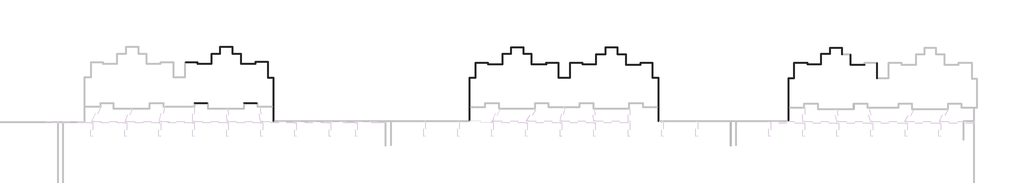
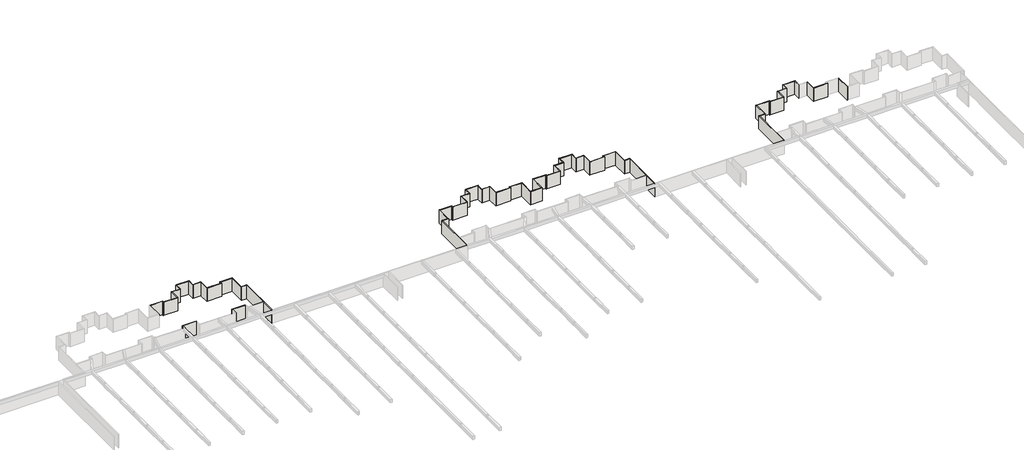
# One storey, part 8 of 16: 67 walls.
"""IFC4 building model written with IfcOpenShell, lengths in millimetres."""

from ifc_helpers import new_model, si_unit, origin, place, context, project, spatial, faceted_brep, element, save

model = new_model("IFC4")

# Units and contexts
model_context = context("Model", 3, world=origin())
ifc_project = project(units=[si_unit("LENGTHUNIT", "METRE", prefix="MILLI")], contexts=[model_context])

# Site, building, storey
site = spatial("IfcSite", under=ifc_project)
building = spatial("IfcBuilding", under=site)
storey = spatial("IfcBuildingStorey", under=building, Name="户型图", Elevation=0.0)

# Walls
placement = place(None, origin())
element("IfcWall", 1, ObjectType="所有墙体", at=placement, inside=storey, context=model_context, shape_type="Brep", body=[
    faceted_brep([(284876.4528769, -118416.941108, 0.0), (287760.8066191, -118416.941108, 0.0), (287880.8066191, -118416.941108, 0.0), (287880.8066191, -118416.941108, 3300.0), (287760.8066191, -118416.941108, 3300.0), (284876.4528769, -118416.941108, 3300.0), (284876.4528769, -118296.941108, 0.0), (284876.4528769, -118296.941108, 3300.0), (287880.8066191, -118296.941108, 3300.0), (287880.8066191, -118296.941108, 0.0)], [[[0, 1, 2, 3, 4, 5]], [[6, 7, 8, 9]], [[2, 1, 0, 6, 9]], [[5, 4, 3, 8, 7]], [[0, 5, 7, 6]], [[3, 2, 9, 8]]]),
])
element("IfcWall", 2, ObjectType="所有墙体", at=placement, inside=storey, context=model_context, shape_type="Brep", body=[
    faceted_brep([(287760.8066191, -118416.941108, 0.0), (287760.8066191, -118816.941108, 0.0), (287760.8066191, -118816.941108, 3300.0), (287760.8066191, -118416.941108, 3300.0), (287880.8066191, -118416.941108, 0.0), (287880.8066191, -118416.941108, 3300.0), (287880.8066191, -118696.941108, 3300.0), (287880.8066191, -118816.941108, 3300.0), (287880.8066191, -118816.941108, 0.0), (287880.8066191, -118696.941108, 0.0)], [[[0, 1, 2, 3]], [[4, 5, 6, 7, 8, 9]], [[1, 0, 4, 9, 8]], [[3, 2, 7, 6, 5]], [[0, 3, 5, 4]], [[2, 1, 8, 7]]]),
])
element("IfcWall", 3, ObjectType="所有墙体", at=placement, inside=storey, context=model_context, shape_type="Brep", body=[
    faceted_brep([(287880.8066191, -118816.941108, 0.0), (291180.8066191, -118816.941108, 0.0), (291180.8066191, -118816.941108, 3300.0), (287880.8066191, -118816.941108, 3300.0), (287880.8066191, -118696.941108, 0.0), (287880.8066191, -118696.941108, 3300.0), (291060.8066191, -118696.941108, 3300.0), (291180.8066191, -118696.941108, 3300.0), (291180.8066191, -118696.941108, 0.0), (291060.8066191, -118696.941108, 0.0)], [[[0, 1, 2, 3]], [[4, 5, 6, 7, 8, 9]], [[1, 0, 4, 9, 8]], [[3, 2, 7, 6, 5]], [[0, 3, 5, 4]], [[2, 1, 8, 7]]]),
])
element("IfcWall", 4, ObjectType="所有墙体", at=placement, inside=storey, context=model_context, shape_type="Brep", body=[
    faceted_brep([(291180.8066191, -118696.941108, 0.0), (291180.8066191, -116445.7855832, 0.0), (291180.8066191, -116325.7855832, 0.0), (291180.8066191, -116325.7855832, 3300.0), (291180.8066191, -116445.7855832, 3300.0), (291180.8066191, -118696.941108, 3300.0), (291060.8066191, -118696.941108, 0.0), (291060.8066191, -118696.941108, 3300.0), (291060.8066191, -116325.7855832, 3300.0), (291060.8066191, -116325.7855832, 0.0)], [[[0, 1, 2, 3, 4, 5]], [[6, 7, 8, 9]], [[2, 1, 0, 6, 9]], [[5, 4, 3, 8, 7]], [[0, 5, 7, 6]], [[3, 2, 9, 8]]]),
])
element("IfcWall", 5, ObjectType="所有墙体", at=placement, inside=storey, context=model_context, shape_type="Brep", body=[
    faceted_brep([(291180.8066191, -116445.7855832, 0.0), (293131.8379904, -116445.7855832, 0.0), (293131.8379904, -116445.7855832, 3300.0), (291180.8066191, -116445.7855832, 3300.0), (291180.8066191, -116325.7855832, 0.0), (291180.8066191, -116325.7855832, 3300.0), (293011.8379904, -116325.7855832, 3300.0), (293131.8379904, -116325.7855832, 3300.0), (293131.8379904, -116325.7855832, 0.0), (293011.8379904, -116325.7855832, 0.0)], [[[0, 1, 2, 3]], [[4, 5, 6, 7, 8, 9]], [[1, 0, 4, 9, 8]], [[3, 2, 7, 6, 5]], [[0, 3, 5, 4]], [[2, 1, 8, 7]]]),
])
element("IfcWall", 6, ObjectType="所有墙体", at=placement, inside=storey, context=model_context, shape_type="Brep", body=[
    faceted_brep([(293131.8379904, -116325.7855832, 0.0), (293131.8379904, -114797.9058341, 0.0), (293131.8379904, -114677.9058341, 0.0), (293131.8379904, -114677.9058341, 3300.0), (293131.8379904, -114797.9058341, 3300.0), (293131.8379904, -116325.7855832, 3300.0), (293011.8379904, -116325.7855832, 0.0), (293011.8379904, -116325.7855832, 3300.0), (293011.8379904, -114677.9058341, 3300.0), (293011.8379904, -114677.9058341, 0.0)], [[[0, 1, 2, 3, 4, 5]], [[6, 7, 8, 9]], [[2, 1, 0, 6, 9]], [[5, 4, 3, 8, 7]], [[0, 5, 7, 6]], [[3, 2, 9, 8]]]),
])
element("IfcWall", 7, ObjectType="所有墙体", at=placement, inside=storey, context=model_context, shape_type="Brep", body=[
    faceted_brep([(293131.8379904, -114797.9058341, 0.0), (296015.4082377, -114797.9058341, 0.0), (296135.4082377, -114797.9058341, 0.0), (296135.4082377, -114797.9058341, 3300.0), (296015.4082377, -114797.9058341, 3300.0), (293131.8379904, -114797.9058341, 3300.0), (293131.8379904, -114677.9058341, 0.0), (293131.8379904, -114677.9058341, 3300.0), (296135.4082377, -114677.9058341, 3300.0), (296135.4082377, -114677.9058341, 0.0)], [[[0, 1, 2, 3, 4, 5]], [[6, 7, 8, 9]], [[2, 1, 0, 6, 9]], [[5, 4, 3, 8, 7]], [[0, 5, 7, 6]], [[3, 2, 9, 8]]]),
])
element("IfcWall", 8, ObjectType="所有墙体", at=placement, inside=storey, context=model_context, shape_type="Brep", body=[
    faceted_brep([(296015.4082377, -114797.9058341, 0.0), (296015.4082377, -116445.7855832, 0.0), (296015.4082377, -116445.7855832, 3300.0), (296015.4082377, -114797.9058341, 3300.0), (296135.4082377, -114797.9058341, 0.0), (296135.4082377, -114797.9058341, 3300.0), (296135.4082377, -116325.7855832, 3300.0), (296135.4082377, -116445.7855832, 3300.0), (296135.4082377, -116445.7855832, 0.0), (296135.4082377, -116325.7855832, 0.0)], [[[0, 1, 2, 3]], [[4, 5, 6, 7, 8, 9]], [[1, 0, 4, 9, 8]], [[3, 2, 7, 6, 5]], [[0, 3, 5, 4]], [[2, 1, 8, 7]]]),
])
element("IfcWall", 9, ObjectType="所有墙体", at=placement, inside=storey, context=model_context, shape_type="Brep", body=[
    faceted_brep([(296135.4082377, -116445.7855832, 0.0), (297963.5984224, -116445.7855832, 0.0), (298083.5984224, -116445.7855832, 0.0), (298083.5984224, -116445.7855832, 3300.0), (297963.5984224, -116445.7855832, 3300.0), (296135.4082377, -116445.7855832, 3300.0), (296135.4082377, -116325.7855832, 0.0), (296135.4082377, -116325.7855832, 3300.0), (298083.5984224, -116325.7855832, 3300.0), (298083.5984224, -116325.7855832, 0.0)], [[[0, 1, 2, 3, 4, 5]], [[6, 7, 8, 9]], [[2, 1, 0, 6, 9]], [[5, 4, 3, 8, 7]], [[0, 5, 7, 6]], [[3, 2, 9, 8]]]),
])
element("IfcWall", 10, ObjectType="所有墙体", at=placement, inside=storey, context=model_context, shape_type="Brep", body=[
    faceted_brep([(297963.5984224, -116445.7855832, 0.0), (297963.5984224, -118816.941108, 0.0), (297963.5984224, -118816.941108, 3300.0), (297963.5984224, -116445.7855832, 3300.0), (298083.5984224, -116445.7855832, 0.0), (298083.5984224, -116445.7855832, 3300.0), (298083.5984224, -118696.941108, 3300.0), (298083.5984224, -118816.941108, 3300.0), (298083.5984224, -118816.941108, 0.0), (298083.5984224, -118696.941108, 0.0)], [[[0, 1, 2, 3]], [[4, 5, 6, 7, 8, 9]], [[1, 0, 4, 9, 8]], [[3, 2, 7, 6, 5]], [[0, 3, 5, 4]], [[2, 1, 8, 7]]]),
])
element("IfcWall", 11, ObjectType="所有墙体", at=placement, inside=storey, context=model_context, shape_type="Brep", body=[
    faceted_brep([(298083.5984224, -118816.941108, 0.0), (301529.8215191, -118816.941108, 0.0), (301529.8215191, -118816.941108, 3300.0), (298083.5984224, -118816.941108, 3300.0), (298083.5984224, -118696.941108, 0.0), (298083.5984224, -118696.941108, 3300.0), (301409.8215191, -118696.941108, 3300.0), (301529.8215191, -118696.941108, 3300.0), (301529.8215191, -118696.941108, 0.0), (301409.8215191, -118696.941108, 0.0)], [[[0, 1, 2, 3]], [[4, 5, 6, 7, 8, 9]], [[1, 0, 4, 9, 8]], [[3, 2, 7, 6, 5]], [[0, 3, 5, 4]], [[2, 1, 8, 7]]]),
])
element("IfcWall", 12, ObjectType="所有墙体", at=placement, inside=storey, context=model_context, shape_type="Brep", body=[
    faceted_brep([(301529.8215191, -118696.941108, 0.0), (301529.8215191, -118356.9724016, 0.0), (301529.8215191, -118236.9724016, 0.0), (301529.8215191, -118236.9724016, 3300.0), (301529.8215191, -118356.9724016, 3300.0), (301529.8215191, -118696.941108, 3300.0), (301409.8215191, -118696.941108, 0.0), (301409.8215191, -118696.941108, 3300.0), (301409.8215191, -118236.9724016, 3300.0), (301409.8215191, -118236.9724016, 0.0)], [[[0, 1, 2, 3, 4, 5]], [[6, 7, 8, 9]], [[2, 1, 0, 6, 9]], [[5, 4, 3, 8, 7]], [[0, 5, 7, 6]], [[3, 2, 9, 8]]]),
])
element("IfcWall", 13, ObjectType="所有墙体", at=placement, inside=storey, context=model_context, shape_type="Brep", body=[
    faceted_brep([(301529.8215191, -118356.9724016, 0.0), (304309.8215191, -118356.9724016, 0.0), (304429.8215191, -118356.9724016, 0.0), (304429.8215191, -118356.9724016, 3300.0), (304309.8215191, -118356.9724016, 3300.0), (301529.8215191, -118356.9724016, 3300.0), (301529.8215191, -118236.9724016, 0.0), (301529.8215191, -118236.9724016, 3300.0), (304429.8215191, -118236.9724016, 3300.0), (304429.8215191, -118236.9724016, 0.0)], [[[0, 1, 2, 3, 4, 5]], [[6, 7, 8, 9]], [[2, 1, 0, 6, 9]], [[5, 4, 3, 8, 7]], [[0, 5, 7, 6]], [[3, 2, 9, 8]]]),
])
element("IfcWall", 14, ObjectType="所有墙体", at=placement, inside=storey, context=model_context, shape_type="Brep", body=[
    faceted_brep([(304309.8215191, -118356.9724016, 0.0), (304309.8215191, -122060.8246701, 0.0), (304309.8215191, -122060.8246701, 3300.0), (304309.8215191, -118356.9724016, 3300.0), (304429.8215191, -118356.9724016, 0.0), (304429.8215191, -118356.9724016, 3300.0), (304429.8215191, -121940.8246701, 3300.0), (304429.8215191, -122060.8246701, 3300.0), (304429.8215191, -122060.8246701, 0.0), (304429.8215191, -121940.8246701, 0.0)], [[[0, 1, 2, 3]], [[4, 5, 6, 7, 8, 9]], [[1, 0, 4, 9, 8]], [[3, 2, 7, 6, 5]], [[0, 3, 5, 4]], [[2, 1, 8, 7]]]),
])
element("IfcWall", 15, ObjectType="所有墙体", at=placement, inside=storey, context=model_context, shape_type="Brep", body=[
    faceted_brep([(304429.8215191, -122060.8246701, 0.0), (305606.5285699, -122060.8246701, 0.0), (305726.5285699, -122060.8246701, 0.0), (305726.5285699, -122060.8246701, 3300.0), (305606.5285699, -122060.8246701, 3300.0), (304429.8215191, -122060.8246701, 3300.0), (304429.8215191, -121940.8246701, 0.0), (304429.8215191, -121940.8246701, 3300.0), (305726.5285699, -121940.8246701, 3300.0), (305726.5285699, -121940.8246701, 0.0)], [[[0, 1, 2, 3, 4, 5]], [[6, 7, 8, 9]], [[2, 1, 0, 6, 9]], [[5, 4, 3, 8, 7]], [[0, 5, 7, 6]], [[3, 2, 9, 8]]]),
])
element("IfcWall", 16, ObjectType="所有墙体", at=placement, inside=storey, context=model_context, shape_type="Brep", body=[
    faceted_brep([(305606.5285699, -122060.8246701, 0.0), (305606.5285699, -128840.8246701, 0.0), (305606.5285699, -128960.8246701, 0.0), (305606.5285699, -132365.1471774, 0.0), (305606.5285699, -132365.1471774, 3300.0), (305606.5285699, -128960.8246701, 3300.0), (305606.5285699, -128840.8246701, 3300.0), (305606.5285699, -122060.8246701, 3300.0), (305726.5285699, -122060.8246701, 0.0), (305726.5285699, -122060.8246701, 3300.0), (305726.5285699, -132245.1471774, 3300.0), (305726.5285699, -132365.1471774, 3300.0), (305726.5285699, -132365.1471774, 0.0), (305726.5285699, -132245.1471774, 0.0)], [[[0, 1, 2, 3, 4, 5, 6, 7]], [[8, 9, 10, 11, 12, 13]], [[3, 2, 1, 0, 8, 13, 12]], [[7, 6, 5, 4, 11, 10, 9]], [[0, 7, 9, 8]], [[4, 3, 12, 11]]]),
])
element("IfcWall", 17, ObjectType="所有墙体", at=placement, inside=storey, context=model_context, shape_type="Brep", body=[
    faceted_brep([(301899.0558962, -127937.9986276, 0.0), (298699.7203632, -127937.9986276, 0.0), (298699.7203632, -127937.9986276, 3300.0), (301899.0558962, -127937.9986276, 3300.0), (301899.0558962, -128057.9986276, 0.0), (301899.0558962, -128057.9986276, 3300.0), (298819.7203632, -128057.9986276, 3300.0), (298699.7203632, -128057.9986276, 3300.0), (298699.7203632, -128057.9986276, 0.0), (298819.7203632, -128057.9986276, 0.0)], [[[0, 1, 2, 3]], [[4, 5, 6, 7, 8, 9]], [[1, 0, 4, 9, 8]], [[3, 2, 7, 6, 5]], [[0, 3, 5, 4]], [[2, 1, 8, 7]]]),
])
element("IfcWall", 18, ObjectType="所有墙体", at=placement, inside=storey, context=model_context, shape_type="Brep", body=[
    faceted_brep([(290199.7203632, -127937.9986276, 0.0), (286999.7203632, -127937.9986276, 0.0), (286999.7203632, -127937.9986276, 3300.0), (290199.7203632, -127937.9986276, 3300.0), (290199.7203632, -128057.9986276, 0.0), (290199.7203632, -128057.9986276, 3300.0), (287119.7203632, -128057.9986276, 3300.0), (286999.7203632, -128057.9986276, 3300.0), (286999.7203632, -128057.9986276, 0.0), (287119.7203632, -128057.9986276, 0.0)], [[[0, 1, 2, 3]], [[4, 5, 6, 7, 8, 9]], [[1, 0, 4, 9, 8]], [[3, 2, 7, 6, 5]], [[0, 3, 5, 4]], [[2, 1, 8, 7]]]),
])
element("IfcWall", 19, ObjectType="所有墙体", at=placement, inside=storey, context=model_context, shape_type="Brep", body=[
    faceted_brep([(351926.5285699, -132245.1471774, 0.0), (351926.5285699, -129061.8026441, 0.0), (351926.5285699, -128941.8026441, 0.0), (351926.5285699, -122163.6737093, 0.0), (351926.5285699, -122043.6737093, 0.0), (351926.5285699, -122043.6737093, 3300.0), (351926.5285699, -122163.6737093, 3300.0), (351926.5285699, -128941.8026441, 3300.0), (351926.5285699, -129061.8026441, 3300.0), (351926.5285699, -132245.1471774, 3300.0), (351806.5285699, -132245.1471774, 0.0), (351806.5285699, -132245.1471774, 3300.0), (351806.5285699, -122043.6737093, 3300.0), (351806.5285699, -122043.6737093, 0.0)], [[[0, 1, 2, 3, 4, 5, 6, 7, 8, 9]], [[10, 11, 12, 13]], [[4, 3, 2, 1, 0, 10, 13]], [[9, 8, 7, 6, 5, 12, 11]], [[0, 9, 11, 10]], [[5, 4, 13, 12]]]),
])
element("IfcWall", 20, ObjectType="所有墙体", at=placement, inside=storey, context=model_context, shape_type="Brep", body=[
    faceted_brep([(351926.5285699, -122163.6737093, 0.0), (353325.4760392, -122163.6737093, 0.0), (353325.4760392, -122163.6737093, 3300.0), (351926.5285699, -122163.6737093, 3300.0), (351926.5285699, -122043.6737093, 0.0), (351926.5285699, -122043.6737093, 3300.0), (353205.4760392, -122043.6737093, 3300.0), (353325.4760392, -122043.6737093, 3300.0), (353325.4760392, -122043.6737093, 0.0), (353205.4760392, -122043.6737093, 0.0)], [[[0, 1, 2, 3]], [[4, 5, 6, 7, 8, 9]], [[1, 0, 4, 9, 8]], [[3, 2, 7, 6, 5]], [[0, 3, 5, 4]], [[2, 1, 8, 7]]]),
])
element("IfcWall", 21, ObjectType="所有墙体", at=placement, inside=storey, context=model_context, shape_type="Brep", body=[
    faceted_brep([(353325.4760392, -122043.6737093, 0.0), (353325.4760392, -118565.1824184, 0.0), (353325.4760392, -118445.1824184, 0.0), (353325.4760392, -118445.1824184, 3300.0), (353325.4760392, -118565.1824184, 3300.0), (353325.4760392, -122043.6737093, 3300.0), (353205.4760392, -122043.6737093, 0.0), (353205.4760392, -122043.6737093, 3300.0), (353205.4760392, -118445.1824184, 3300.0), (353205.4760392, -118445.1824184, 0.0)], [[[0, 1, 2, 3, 4, 5]], [[6, 7, 8, 9]], [[2, 1, 0, 6, 9]], [[5, 4, 3, 8, 7]], [[0, 5, 7, 6]], [[3, 2, 9, 8]]]),
])
element("IfcWall", 22, ObjectType="所有墙体", at=placement, inside=storey, context=model_context, shape_type="Brep", body=[
    faceted_brep([(353325.4760392, -118565.1824184, 0.0), (356109.6030574, -118565.1824184, 0.0), (356229.6030574, -118565.1824184, 0.0), (356229.6030574, -118565.1824184, 3300.0), (356109.6030574, -118565.1824184, 3300.0), (353325.4760392, -118565.1824184, 3300.0), (353325.4760392, -118445.1824184, 0.0), (353325.4760392, -118445.1824184, 3300.0), (356229.6030574, -118445.1824184, 3300.0), (356229.6030574, -118445.1824184, 0.0)], [[[0, 1, 2, 3, 4, 5]], [[6, 7, 8, 9]], [[2, 1, 0, 6, 9]], [[5, 4, 3, 8, 7]], [[0, 5, 7, 6]], [[3, 2, 9, 8]]]),
])
element("IfcWall", 23, ObjectType="所有墙体", at=placement, inside=storey, context=model_context, shape_type="Brep", body=[
    faceted_brep([(356109.6030574, -118565.1824184, 0.0), (356109.6030574, -118916.8002474, 0.0), (356109.6030574, -118916.8002474, 3300.0), (356109.6030574, -118565.1824184, 3300.0), (356229.6030574, -118565.1824184, 0.0), (356229.6030574, -118565.1824184, 3300.0), (356229.6030574, -118796.8002474, 3300.0), (356229.6030574, -118916.8002474, 3300.0), (356229.6030574, -118916.8002474, 0.0), (356229.6030574, -118796.8002474, 0.0)], [[[0, 1, 2, 3]], [[4, 5, 6, 7, 8, 9]], [[1, 0, 4, 9, 8]], [[3, 2, 7, 6, 5]], [[0, 3, 5, 4]], [[2, 1, 8, 7]]]),
])
element("IfcWall", 24, ObjectType="所有墙体", at=placement, inside=storey, context=model_context, shape_type="Brep", body=[
    faceted_brep([(356229.6030574, -118916.8002474, 0.0), (359629.1545604, -118916.8002474, 0.0), (359629.1545604, -118916.8002474, 3300.0), (356229.6030574, -118916.8002474, 3300.0), (356229.6030574, -118796.8002474, 0.0), (356229.6030574, -118796.8002474, 3300.0), (359509.1545604, -118796.8002474, 3300.0), (359629.1545604, -118796.8002474, 3300.0), (359629.1545604, -118796.8002474, 0.0), (359509.1545604, -118796.8002474, 0.0)], [[[0, 1, 2, 3]], [[4, 5, 6, 7, 8, 9]], [[1, 0, 4, 9, 8]], [[3, 2, 7, 6, 5]], [[0, 3, 5, 4]], [[2, 1, 8, 7]]]),
])
element("IfcWall", 25, ObjectType="所有墙体", at=placement, inside=storey, context=model_context, shape_type="Brep", body=[
    faceted_brep([(359629.1545604, -118796.8002474, 0.0), (359629.1545604, -116522.0993217, 0.0), (359629.1545604, -116402.0993217, 0.0), (359629.1545604, -116402.0993217, 3300.0), (359629.1545604, -116522.0993217, 3300.0), (359629.1545604, -118796.8002474, 3300.0), (359509.1545604, -118796.8002474, 0.0), (359509.1545604, -118796.8002474, 3300.0), (359509.1545604, -116402.0993217, 3300.0), (359509.1545604, -116402.0993217, 0.0)], [[[0, 1, 2, 3, 4, 5]], [[6, 7, 8, 9]], [[2, 1, 0, 6, 9]], [[5, 4, 3, 8, 7]], [[0, 5, 7, 6]], [[3, 2, 9, 8]]]),
])
element("IfcWall", 26, ObjectType="所有墙体", at=placement, inside=storey, context=model_context, shape_type="Brep", body=[
    faceted_brep([(359629.1545604, -116522.0993217, 0.0), (361632.0016702, -116522.0993217, 0.0), (361632.0016702, -116522.0993217, 3300.0), (359629.1545604, -116522.0993217, 3300.0), (359629.1545604, -116402.0993217, 0.0), (359629.1545604, -116402.0993217, 3300.0), (361512.0016702, -116402.0993217, 3300.0), (361632.0016702, -116402.0993217, 3300.0), (361632.0016702, -116402.0993217, 0.0), (361512.0016702, -116402.0993217, 0.0)], [[[0, 1, 2, 3]], [[4, 5, 6, 7, 8, 9]], [[1, 0, 4, 9, 8]], [[3, 2, 7, 6, 5]], [[0, 3, 5, 4]], [[2, 1, 8, 7]]]),
])
element("IfcWall", 27, ObjectType="所有墙体", at=placement, inside=storey, context=model_context, shape_type="Brep", body=[
    faceted_brep([(361632.0016702, -116402.0993217, 0.0), (361632.0016702, -114974.4465118, 0.0), (361632.0016702, -114854.4465118, 0.0), (361632.0016702, -114854.4465118, 3300.0), (361632.0016702, -114974.4465118, 3300.0), (361632.0016702, -116402.0993217, 3300.0), (361512.0016702, -116402.0993217, 0.0), (361512.0016702, -116402.0993217, 3300.0), (361512.0016702, -114854.4465118, 3300.0), (361512.0016702, -114854.4465118, 0.0)], [[[0, 1, 2, 3, 4, 5]], [[6, 7, 8, 9]], [[2, 1, 0, 6, 9]], [[5, 4, 3, 8, 7]], [[0, 5, 7, 6]], [[3, 2, 9, 8]]]),
])
element("IfcWall", 28, ObjectType="所有墙体", at=placement, inside=storey, context=model_context, shape_type="Brep", body=[
    faceted_brep([(361632.0016702, -114974.4465118, 0.0), (364414.5113757, -114974.4465118, 0.0), (364534.5113757, -114974.4465118, 0.0), (364534.5113757, -114974.4465118, 3300.0), (364414.5113757, -114974.4465118, 3300.0), (361632.0016702, -114974.4465118, 3300.0), (361632.0016702, -114854.4465118, 0.0), (361632.0016702, -114854.4465118, 3300.0), (364534.5113757, -114854.4465118, 3300.0), (364534.5113757, -114854.4465118, 0.0)], [[[0, 1, 2, 3, 4, 5]], [[6, 7, 8, 9]], [[2, 1, 0, 6, 9]], [[5, 4, 3, 8, 7]], [[0, 5, 7, 6]], [[3, 2, 9, 8]]]),
])
element("IfcWall", 29, ObjectType="所有墙体", at=placement, inside=storey, context=model_context, shape_type="Brep", body=[
    faceted_brep([(364414.5113757, -114974.4465118, 0.0), (364414.5113757, -116522.0993217, 0.0), (364414.5113757, -116522.0993217, 3300.0), (364414.5113757, -114974.4465118, 3300.0), (364534.5113757, -114974.4465118, 0.0), (364534.5113757, -114974.4465118, 3300.0), (364534.5113757, -116402.0993217, 3300.0), (364534.5113757, -116522.0993217, 3300.0), (364534.5113757, -116522.0993217, 0.0), (364534.5113757, -116402.0993217, 0.0)], [[[0, 1, 2, 3]], [[4, 5, 6, 7, 8, 9]], [[1, 0, 4, 9, 8]], [[3, 2, 7, 6, 5]], [[0, 3, 5, 4]], [[2, 1, 8, 7]]]),
])
element("IfcWall", 30, ObjectType="所有墙体", at=placement, inside=storey, context=model_context, shape_type="Brep", body=[
    faceted_brep([(364534.5113757, -116522.0993217, 0.0), (366311.8284806, -116522.0993217, 0.0), (366431.8284806, -116522.0993217, 0.0), (366431.8284806, -116522.0993217, 3300.0), (366311.8284806, -116522.0993217, 3300.0), (364534.5113757, -116522.0993217, 3300.0), (364534.5113757, -116402.0993217, 0.0), (364534.5113757, -116402.0993217, 3300.0), (366431.8284806, -116402.0993217, 3300.0), (366431.8284806, -116402.0993217, 0.0)], [[[0, 1, 2, 3, 4, 5]], [[6, 7, 8, 9]], [[2, 1, 0, 6, 9]], [[5, 4, 3, 8, 7]], [[0, 5, 7, 6]], [[3, 2, 9, 8]]]),
])
element("IfcWall", 31, ObjectType="所有墙体", at=placement, inside=storey, context=model_context, shape_type="Brep", body=[
    faceted_brep([(366311.8284806, -116522.0993217, 0.0), (366311.8284806, -118916.8002474, 0.0), (366311.8284806, -118916.8002474, 3300.0), (366311.8284806, -116522.0993217, 3300.0), (366431.8284806, -116522.0993217, 0.0), (366431.8284806, -116522.0993217, 3300.0), (366431.8284806, -118796.8002474, 3300.0), (366431.8284806, -118916.8002474, 3300.0), (366431.8284806, -118916.8002474, 0.0), (366431.8284806, -118796.8002474, 0.0)], [[[0, 1, 2, 3]], [[4, 5, 6, 7, 8, 9]], [[1, 0, 4, 9, 8]], [[3, 2, 7, 6, 5]], [[0, 3, 5, 4]], [[2, 1, 8, 7]]]),
])
element("IfcWall", 32, ObjectType="所有墙体", at=placement, inside=storey, context=model_context, shape_type="Brep", body=[
    faceted_brep([(366431.8284806, -118916.8002474, 0.0), (369929.0923666, -118916.8002474, 0.0), (369929.0923666, -118916.8002474, 3300.0), (366431.8284806, -118916.8002474, 3300.0), (366431.8284806, -118796.8002474, 0.0), (366431.8284806, -118796.8002474, 3300.0), (369809.0923666, -118796.8002474, 3300.0), (369929.0923666, -118796.8002474, 3300.0), (369929.0923666, -118796.8002474, 0.0), (369809.0923666, -118796.8002474, 0.0)], [[[0, 1, 2, 3]], [[4, 5, 6, 7, 8, 9]], [[1, 0, 4, 9, 8]], [[3, 2, 7, 6, 5]], [[0, 3, 5, 4]], [[2, 1, 8, 7]]]),
])
element("IfcWall", 33, ObjectType="所有墙体", at=placement, inside=storey, context=model_context, shape_type="Brep", body=[
    faceted_brep([(369929.0923666, -118796.8002474, 0.0), (369929.0923666, -118565.1824184, 0.0), (369929.0923666, -118445.1824184, 0.0), (369929.0923666, -118445.1824184, 3300.0), (369929.0923666, -118565.1824184, 3300.0), (369929.0923666, -118796.8002474, 3300.0), (369809.0923666, -118796.8002474, 0.0), (369809.0923666, -118796.8002474, 3300.0), (369809.0923666, -118445.1824184, 3300.0), (369809.0923666, -118445.1824184, 0.0)], [[[0, 1, 2, 3, 4, 5]], [[6, 7, 8, 9]], [[2, 1, 0, 6, 9]], [[5, 4, 3, 8, 7]], [[0, 5, 7, 6]], [[3, 2, 9, 8]]]),
])
element("IfcWall", 34, ObjectType="所有墙体", at=placement, inside=storey, context=model_context, shape_type="Brep", body=[
    faceted_brep([(369929.0923666, -118565.1824184, 0.0), (372659.6169578, -118565.1824184, 0.0), (372779.6169578, -118565.1824184, 0.0), (372779.6169578, -118565.1824184, 3300.0), (372659.6169578, -118565.1824184, 3300.0), (369929.0923666, -118565.1824184, 3300.0), (369929.0923666, -118445.1824184, 0.0), (369929.0923666, -118445.1824184, 3300.0), (372779.6169578, -118445.1824184, 3300.0), (372779.6169578, -118445.1824184, 0.0)], [[[0, 1, 2, 3, 4, 5]], [[6, 7, 8, 9]], [[2, 1, 0, 6, 9]], [[5, 4, 3, 8, 7]], [[0, 5, 7, 6]], [[3, 2, 9, 8]]]),
])
element("IfcWall", 35, ObjectType="所有墙体", at=placement, inside=storey, context=model_context, shape_type="Brep", body=[
    faceted_brep([(372659.6169578, -118565.1824184, 0.0), (372659.6169578, -122136.8888457, 0.0), (372659.6169578, -122136.8888457, 3300.0), (372659.6169578, -118565.1824184, 3300.0), (372779.6169578, -118565.1824184, 0.0), (372779.6169578, -118565.1824184, 3300.0), (372779.6169578, -122016.8888457, 3300.0), (372779.6169578, -122136.8888457, 3300.0), (372779.6169578, -122136.8888457, 0.0), (372779.6169578, -122016.8888457, 0.0)], [[[0, 1, 2, 3]], [[4, 5, 6, 7, 8, 9]], [[1, 0, 4, 9, 8]], [[3, 2, 7, 6, 5]], [[0, 3, 5, 4]], [[2, 1, 8, 7]]]),
])
element("IfcWall", 36, ObjectType="所有墙体", at=placement, inside=storey, context=model_context, shape_type="Brep", body=[
    faceted_brep([(372779.6169578, -122136.8888457, 0.0), (375475.6329816, -122136.8888457, 0.0), (375475.6329816, -122136.8888457, 3300.0), (372779.6169578, -122136.8888457, 3300.0), (372779.6169578, -122016.8888457, 0.0), (372779.6169578, -122016.8888457, 3300.0), (375355.6329816, -122016.8888457, 3300.0), (375475.6329816, -122016.8888457, 3300.0), (375475.6329816, -122016.8888457, 0.0), (375355.6329816, -122016.8888457, 0.0)], [[[0, 1, 2, 3]], [[4, 5, 6, 7, 8, 9]], [[1, 0, 4, 9, 8]], [[3, 2, 7, 6, 5]], [[0, 3, 5, 4]], [[2, 1, 8, 7]]]),
])
element("IfcWall", 37, ObjectType="所有墙体", at=placement, inside=storey, context=model_context, shape_type="Brep", body=[
    faceted_brep([(375475.6329816, -122016.8888457, 0.0), (375475.6329816, -118565.1824184, 0.0), (375475.6329816, -118445.1824184, 0.0), (375475.6329816, -118445.1824184, 3300.0), (375475.6329816, -118565.1824184, 3300.0), (375475.6329816, -122016.8888457, 3300.0), (375355.6329816, -122016.8888457, 0.0), (375355.6329816, -122016.8888457, 3300.0), (375355.6329816, -118445.1824184, 3300.0), (375355.6329816, -118445.1824184, 0.0)], [[[0, 1, 2, 3, 4, 5]], [[6, 7, 8, 9]], [[2, 1, 0, 6, 9]], [[5, 4, 3, 8, 7]], [[0, 5, 7, 6]], [[3, 2, 9, 8]]]),
])
element("IfcWall", 38, ObjectType="所有墙体", at=placement, inside=storey, context=model_context, shape_type="Brep", body=[
    faceted_brep([(375475.6329816, -118565.1824184, 0.0), (378359.9551511, -118565.1824184, 0.0), (378479.9551511, -118565.1824184, 0.0), (378479.9551511, -118565.1824184, 3300.0), (378359.9551511, -118565.1824184, 3300.0), (375475.6329816, -118565.1824184, 3300.0), (375475.6329816, -118445.1824184, 0.0), (375475.6329816, -118445.1824184, 3300.0), (378479.9551511, -118445.1824184, 3300.0), (378479.9551511, -118445.1824184, 0.0)], [[[0, 1, 2, 3, 4, 5]], [[6, 7, 8, 9]], [[2, 1, 0, 6, 9]], [[5, 4, 3, 8, 7]], [[0, 5, 7, 6]], [[3, 2, 9, 8]]]),
])
element("IfcWall", 39, ObjectType="所有墙体", at=placement, inside=storey, context=model_context, shape_type="Brep", body=[
    faceted_brep([(378359.9551511, -118565.1824184, 0.0), (378359.9551511, -118916.8002474, 0.0), (378359.9551511, -118916.8002474, 3300.0), (378359.9551511, -118565.1824184, 3300.0), (378479.9551511, -118565.1824184, 0.0), (378479.9551511, -118565.1824184, 3300.0), (378479.9551511, -118796.8002474, 3300.0), (378479.9551511, -118916.8002474, 3300.0), (378479.9551511, -118916.8002474, 0.0), (378479.9551511, -118796.8002474, 0.0)], [[[0, 1, 2, 3]], [[4, 5, 6, 7, 8, 9]], [[1, 0, 4, 9, 8]], [[3, 2, 7, 6, 5]], [[0, 3, 5, 4]], [[2, 1, 8, 7]]]),
])
element("IfcWall", 40, ObjectType="所有墙体", at=placement, inside=storey, context=model_context, shape_type="Brep", body=[
    faceted_brep([(378479.9551511, -118916.8002474, 0.0), (381679.4198272, -118916.8002474, 0.0), (381679.4198272, -118916.8002474, 3300.0), (378479.9551511, -118916.8002474, 3300.0), (378479.9551511, -118796.8002474, 0.0), (378479.9551511, -118796.8002474, 3300.0), (381559.4198272, -118796.8002474, 3300.0), (381679.4198272, -118796.8002474, 3300.0), (381679.4198272, -118796.8002474, 0.0), (381559.4198272, -118796.8002474, 0.0)], [[[0, 1, 2, 3]], [[4, 5, 6, 7, 8, 9]], [[1, 0, 4, 9, 8]], [[3, 2, 7, 6, 5]], [[0, 3, 5, 4]], [[2, 1, 8, 7]]]),
])
element("IfcWall", 41, ObjectType="所有墙体", at=placement, inside=storey, context=model_context, shape_type="Brep", body=[
    faceted_brep([(381679.4198272, -118796.8002474, 0.0), (381679.4198272, -116546.7051282, 0.0), (381679.4198272, -116426.7051282, 0.0), (381679.4198272, -116426.7051282, 3300.0), (381679.4198272, -116546.7051282, 3300.0), (381679.4198272, -118796.8002474, 3300.0), (381559.4198272, -118796.8002474, 0.0), (381559.4198272, -118796.8002474, 3300.0), (381559.4198272, -116426.7051282, 3300.0), (381559.4198272, -116426.7051282, 0.0)], [[[0, 1, 2, 3, 4, 5]], [[6, 7, 8, 9]], [[2, 1, 0, 6, 9]], [[5, 4, 3, 8, 7]], [[0, 5, 7, 6]], [[3, 2, 9, 8]]]),
])
element("IfcWall", 42, ObjectType="所有墙体", at=placement, inside=storey, context=model_context, shape_type="Brep", body=[
    faceted_brep([(381679.4198272, -116546.7051282, 0.0), (383831.9880347, -116546.7051282, 0.0), (383831.9880347, -116546.7051282, 3300.0), (381679.4198272, -116546.7051282, 3300.0), (381679.4198272, -116426.7051282, 0.0), (381679.4198272, -116426.7051282, 3300.0), (383711.9880347, -116426.7051282, 3300.0), (383831.9880347, -116426.7051282, 3300.0), (383831.9880347, -116426.7051282, 0.0), (383711.9880347, -116426.7051282, 0.0)], [[[0, 1, 2, 3]], [[4, 5, 6, 7, 8, 9]], [[1, 0, 4, 9, 8]], [[3, 2, 7, 6, 5]], [[0, 3, 5, 4]], [[2, 1, 8, 7]]]),
])
element("IfcWall", 43, ObjectType="所有墙体", at=placement, inside=storey, context=model_context, shape_type="Brep", body=[
    faceted_brep([(383831.9880347, -116426.7051282, 0.0), (383831.9880347, -114899.0502735, 0.0), (383831.9880347, -114779.0502735, 0.0), (383831.9880347, -114779.0502735, 3300.0), (383831.9880347, -114899.0502735, 3300.0), (383831.9880347, -116426.7051282, 3300.0), (383711.9880347, -116426.7051282, 0.0), (383711.9880347, -116426.7051282, 3300.0), (383711.9880347, -114779.0502735, 3300.0), (383711.9880347, -114779.0502735, 0.0)], [[[0, 1, 2, 3, 4, 5]], [[6, 7, 8, 9]], [[2, 1, 0, 6, 9]], [[5, 4, 3, 8, 7]], [[0, 5, 7, 6]], [[3, 2, 9, 8]]]),
])
element("IfcWall", 44, ObjectType="所有墙体", at=placement, inside=storey, context=model_context, shape_type="Brep", body=[
    faceted_brep([(383831.9880347, -114899.0502735, 0.0), (386614.6093322, -114899.0502735, 0.0), (386734.6093322, -114899.0502735, 0.0), (386734.6093322, -114899.0502735, 3300.0), (386614.6093322, -114899.0502735, 3300.0), (383831.9880347, -114899.0502735, 3300.0), (383831.9880347, -114779.0502735, 0.0), (383831.9880347, -114779.0502735, 3300.0), (386734.6093322, -114779.0502735, 3300.0), (386734.6093322, -114779.0502735, 0.0)], [[[0, 1, 2, 3, 4, 5]], [[6, 7, 8, 9]], [[2, 1, 0, 6, 9]], [[5, 4, 3, 8, 7]], [[0, 5, 7, 6]], [[3, 2, 9, 8]]]),
])
element("IfcWall", 45, ObjectType="所有墙体", at=placement, inside=storey, context=model_context, shape_type="Brep", body=[
    faceted_brep([(386614.6093322, -114899.0502735, 0.0), (386614.6093322, -116546.7051282, 0.0), (386614.6093322, -116546.7051282, 3300.0), (386614.6093322, -114899.0502735, 3300.0), (386734.6093322, -114899.0502735, 0.0), (386734.6093322, -114899.0502735, 3300.0), (386734.6093322, -116426.7051282, 3300.0), (386734.6093322, -116546.7051282, 3300.0), (386734.6093322, -116546.7051282, 0.0), (386734.6093322, -116426.7051282, 0.0)], [[[0, 1, 2, 3]], [[4, 5, 6, 7, 8, 9]], [[1, 0, 4, 9, 8]], [[3, 2, 7, 6, 5]], [[0, 3, 5, 4]], [[2, 1, 8, 7]]]),
])
element("IfcWall", 46, ObjectType="所有墙体", at=placement, inside=storey, context=model_context, shape_type="Brep", body=[
    faceted_brep([(386734.6093322, -116546.7051282, 0.0), (388562.7997606, -116546.7051282, 0.0), (388682.7997606, -116546.7051282, 0.0), (388682.7997606, -116546.7051282, 3300.0), (388562.7997606, -116546.7051282, 3300.0), (386734.6093322, -116546.7051282, 3300.0), (386734.6093322, -116426.7051282, 0.0), (386734.6093322, -116426.7051282, 3300.0), (388682.7997606, -116426.7051282, 3300.0), (388682.7997606, -116426.7051282, 0.0)], [[[0, 1, 2, 3, 4, 5]], [[6, 7, 8, 9]], [[2, 1, 0, 6, 9]], [[5, 4, 3, 8, 7]], [[0, 5, 7, 6]], [[3, 2, 9, 8]]]),
])
element("IfcWall", 47, ObjectType="所有墙体", at=placement, inside=storey, context=model_context, shape_type="Brep", body=[
    faceted_brep([(388562.7997606, -116546.7051282, 0.0), (388562.7997606, -119046.7051282, 0.0), (388562.7997606, -119046.7051282, 3300.0), (388562.7997606, -116546.7051282, 3300.0), (388682.7997606, -116546.7051282, 0.0), (388682.7997606, -116546.7051282, 3300.0), (388682.7997606, -118926.7051282, 3300.0), (388682.7997606, -119046.7051282, 3300.0), (388682.7997606, -119046.7051282, 0.0), (388682.7997606, -118926.7051282, 0.0)], [[[0, 1, 2, 3]], [[4, 5, 6, 7, 8, 9]], [[1, 0, 4, 9, 8]], [[3, 2, 7, 6, 5]], [[0, 3, 5, 4]], [[2, 1, 8, 7]]]),
])
element("IfcWall", 48, ObjectType="所有墙体", at=placement, inside=storey, context=model_context, shape_type="Brep", body=[
    faceted_brep([(388682.7997606, -119046.7051282, 0.0), (392129.0227393, -119046.7051282, 0.0), (392129.0227393, -119046.7051282, 3300.0), (388682.7997606, -119046.7051282, 3300.0), (388682.7997606, -118926.7051282, 0.0), (388682.7997606, -118926.7051282, 3300.0), (392009.0227393, -118926.7051282, 3300.0), (392129.0227393, -118926.7051282, 3300.0), (392129.0227393, -118926.7051282, 0.0), (392009.0227393, -118926.7051282, 0.0)], [[[0, 1, 2, 3]], [[4, 5, 6, 7, 8, 9]], [[1, 0, 4, 9, 8]], [[3, 2, 7, 6, 5]], [[0, 3, 5, 4]], [[2, 1, 8, 7]]]),
])
element("IfcWall", 49, ObjectType="所有墙体", at=placement, inside=storey, context=model_context, shape_type="Brep", body=[
    faceted_brep([(392129.0227393, -118926.7051282, 0.0), (392129.0227393, -118558.3670456, 0.0), (392129.0227393, -118438.3670456, 0.0), (392129.0227393, -118438.3670456, 3300.0), (392129.0227393, -118558.3670456, 3300.0), (392129.0227393, -118926.7051282, 3300.0), (392009.0227393, -118926.7051282, 0.0), (392009.0227393, -118926.7051282, 3300.0), (392009.0227393, -118438.3670456, 3300.0), (392009.0227393, -118438.3670456, 0.0)], [[[0, 1, 2, 3, 4, 5]], [[6, 7, 8, 9]], [[2, 1, 0, 6, 9]], [[5, 4, 3, 8, 7]], [[0, 5, 7, 6]], [[3, 2, 9, 8]]]),
])
element("IfcWall", 50, ObjectType="所有墙体", at=placement, inside=storey, context=model_context, shape_type="Brep", body=[
    faceted_brep([(392129.0227393, -118558.3670456, 0.0), (394860.7541571, -118558.3670456, 0.0), (394980.7541571, -118558.3670456, 0.0), (394980.7541571, -118558.3670456, 3300.0), (394860.7541571, -118558.3670456, 3300.0), (392129.0227393, -118558.3670456, 3300.0), (392129.0227393, -118438.3670456, 0.0), (392129.0227393, -118438.3670456, 3300.0), (394980.7541571, -118438.3670456, 3300.0), (394980.7541571, -118438.3670456, 0.0)], [[[0, 1, 2, 3, 4, 5]], [[6, 7, 8, 9]], [[2, 1, 0, 6, 9]], [[5, 4, 3, 8, 7]], [[0, 5, 7, 6]], [[3, 2, 9, 8]]]),
])
element("IfcWall", 51, ObjectType="所有墙体", at=placement, inside=storey, context=model_context, shape_type="Brep", body=[
    faceted_brep([(394860.7541571, -118558.3670456, 0.0), (394860.7541571, -122161.8026441, 0.0), (394860.7541571, -122161.8026441, 3300.0), (394860.7541571, -118558.3670456, 3300.0), (394980.7541571, -118558.3670456, 0.0), (394980.7541571, -118558.3670456, 3300.0), (394980.7541571, -122041.8026441, 3300.0), (394980.7541571, -122161.8026441, 3300.0), (394980.7541571, -122161.8026441, 0.0), (394980.7541571, -122041.8026441, 0.0)], [[[0, 1, 2, 3]], [[4, 5, 6, 7, 8, 9]], [[1, 0, 4, 9, 8]], [[3, 2, 7, 6, 5]], [[0, 3, 5, 4]], [[2, 1, 8, 7]]]),
])
element("IfcWall", 52, ObjectType="所有墙体", at=placement, inside=storey, context=model_context, shape_type="Brep", body=[
    faceted_brep([(394980.7541571, -122161.8026441, 0.0), (396205.7298502, -122161.8026441, 0.0), (396325.7298502, -122161.8026441, 0.0), (396325.7298502, -122161.8026441, 3300.0), (396205.7298502, -122161.8026441, 3300.0), (394980.7541571, -122161.8026441, 3300.0), (394980.7541571, -122041.8026441, 0.0), (394980.7541571, -122041.8026441, 3300.0), (396325.7298502, -122041.8026441, 3300.0), (396325.7298502, -122041.8026441, 0.0)], [[[0, 1, 2, 3, 4, 5]], [[6, 7, 8, 9]], [[2, 1, 0, 6, 9]], [[5, 4, 3, 8, 7]], [[0, 5, 7, 6]], [[3, 2, 9, 8]]]),
])
element("IfcWall", 53, ObjectType="所有墙体", at=placement, inside=storey, context=model_context, shape_type="Brep", body=[
    faceted_brep([(396205.7298502, -122161.8026441, 0.0), (396205.7298502, -128941.8026441, 0.0), (396205.7298502, -129061.8026441, 0.0), (396205.7298502, -132365.1471775, 0.0), (396205.7298502, -132365.1471775, 3300.0), (396205.7298502, -129061.8026441, 3300.0), (396205.7298502, -128941.8026441, 3300.0), (396205.7298502, -122161.8026441, 3300.0), (396325.7298502, -122161.8026441, 0.0), (396325.7298502, -122161.8026441, 3300.0), (396325.7298502, -132245.1471775, 3300.0), (396325.7298502, -132365.1471775, 3300.0), (396325.7298502, -132365.1471775, 0.0), (396325.7298502, -132245.1471775, 0.0)], [[[0, 1, 2, 3, 4, 5, 6, 7]], [[8, 9, 10, 11, 12, 13]], [[3, 2, 1, 0, 8, 13, 12]], [[7, 6, 5, 4, 11, 10, 9]], [[0, 7, 9, 8]], [[4, 3, 12, 11]]]),
])
element("IfcWall", 54, ObjectType="所有墙体", at=placement, inside=storey, context=model_context, shape_type="Brep", body=[
    faceted_brep([(426925.7298502, -132245.1471775, 0.0), (426925.7298502, -129162.7220843, 0.0), (426925.7298502, -129042.7220843, 0.0), (426925.7298502, -122197.510137, 0.0), (426925.7298502, -122077.510137, 0.0), (426925.7298502, -122077.510137, 3300.0), (426925.7298502, -122197.510137, 3300.0), (426925.7298502, -129042.7220843, 3300.0), (426925.7298502, -129162.7220843, 3300.0), (426925.7298502, -132245.1471775, 3300.0), (426805.7298502, -132245.1471775, 0.0), (426805.7298502, -132245.1471775, 3300.0), (426805.7298502, -122077.510137, 3300.0), (426805.7298502, -122077.510137, 0.0)], [[[0, 1, 2, 3, 4, 5, 6, 7, 8, 9]], [[10, 11, 12, 13]], [[4, 3, 2, 1, 0, 10, 13]], [[9, 8, 7, 6, 5, 12, 11]], [[0, 9, 11, 10]], [[5, 4, 13, 12]]]),
])
element("IfcWall", 55, ObjectType="所有墙体", at=placement, inside=storey, context=model_context, shape_type="Brep", body=[
    faceted_brep([(426925.7298502, -122197.510137, 0.0), (428275.5982085, -122197.510137, 0.0), (428275.5982085, -122197.510137, 3300.0), (426925.7298502, -122197.510137, 3300.0), (426925.7298502, -122077.510137, 0.0), (426925.7298502, -122077.510137, 3300.0), (428155.5982085, -122077.510137, 3300.0), (428275.5982085, -122077.510137, 3300.0), (428275.5982085, -122077.510137, 0.0), (428155.5982085, -122077.510137, 0.0)], [[[0, 1, 2, 3]], [[4, 5, 6, 7, 8, 9]], [[1, 0, 4, 9, 8]], [[3, 2, 7, 6, 5]], [[0, 3, 5, 4]], [[2, 1, 8, 7]]]),
])
element("IfcWall", 56, ObjectType="所有墙体", at=placement, inside=storey, context=model_context, shape_type="Brep", body=[
    faceted_brep([(428275.5982085, -122077.510137, 0.0), (428275.5982085, -118598.8141783, 0.0), (428275.5982085, -118478.8141783, 0.0), (428275.5982085, -118478.8141783, 3300.0), (428275.5982085, -118598.8141783, 3300.0), (428275.5982085, -122077.510137, 3300.0), (428155.5982085, -122077.510137, 0.0), (428155.5982085, -122077.510137, 3300.0), (428155.5982085, -118478.8141783, 3300.0), (428155.5982085, -118478.8141783, 0.0)], [[[0, 1, 2, 3, 4, 5]], [[6, 7, 8, 9]], [[2, 1, 0, 6, 9]], [[5, 4, 3, 8, 7]], [[0, 5, 7, 6]], [[3, 2, 9, 8]]]),
])
element("IfcWall", 57, ObjectType="所有墙体", at=placement, inside=storey, context=model_context, shape_type="Brep", body=[
    faceted_brep([(428275.5982085, -118598.8141783, 0.0), (431259.6159134, -118598.8141783, 0.0), (431379.6159134, -118598.8141783, 0.0), (431379.6159134, -118598.8141783, 3300.0), (431259.6159134, -118598.8141783, 3300.0), (428275.5982085, -118598.8141783, 3300.0), (428275.5982085, -118478.8141783, 0.0), (428275.5982085, -118478.8141783, 3300.0), (431379.6159134, -118478.8141783, 3300.0), (431379.6159134, -118478.8141783, 0.0)], [[[0, 1, 2, 3, 4, 5]], [[6, 7, 8, 9]], [[2, 1, 0, 6, 9]], [[5, 4, 3, 8, 7]], [[0, 5, 7, 6]], [[3, 2, 9, 8]]]),
])
element("IfcWall", 58, ObjectType="所有墙体", at=placement, inside=storey, context=model_context, shape_type="Brep", body=[
    faceted_brep([(431259.6159134, -118598.8141783, 0.0), (431259.6159134, -118902.2781299, 0.0), (431259.6159134, -118902.2781299, 3300.0), (431259.6159134, -118598.8141783, 3300.0), (431379.6159134, -118598.8141783, 0.0), (431379.6159134, -118598.8141783, 3300.0), (431379.6159134, -118782.2781299, 3300.0), (431379.6159134, -118902.2781299, 3300.0), (431379.6159134, -118902.2781299, 0.0), (431379.6159134, -118782.2781299, 0.0)], [[[0, 1, 2, 3]], [[4, 5, 6, 7, 8, 9]], [[1, 0, 4, 9, 8]], [[3, 2, 7, 6, 5]], [[0, 3, 5, 4]], [[2, 1, 8, 7]]]),
])
element("IfcWall", 59, ObjectType="所有墙体", at=placement, inside=storey, context=model_context, shape_type="Brep", body=[
    faceted_brep([(431379.6159134, -118902.2781299, 0.0), (434579.6159134, -118902.2781299, 0.0), (434579.6159134, -118902.2781299, 3300.0), (431379.6159134, -118902.2781299, 3300.0), (431379.6159134, -118782.2781299, 0.0), (431379.6159134, -118782.2781299, 3300.0), (434459.6159134, -118782.2781299, 3300.0), (434579.6159134, -118782.2781299, 3300.0), (434579.6159134, -118782.2781299, 0.0), (434459.6159134, -118782.2781299, 0.0)], [[[0, 1, 2, 3]], [[4, 5, 6, 7, 8, 9]], [[1, 0, 4, 9, 8]], [[3, 2, 7, 6, 5]], [[0, 3, 5, 4]], [[2, 1, 8, 7]]]),
])
element("IfcWall", 60, ObjectType="所有墙体", at=placement, inside=storey, context=model_context, shape_type="Brep", body=[
    faceted_brep([(434579.6159134, -118782.2781299, 0.0), (434579.6159134, -116505.8475066, 0.0), (434579.6159134, -116385.8475066, 0.0), (434579.6159134, -116385.8475066, 3300.0), (434579.6159134, -116505.8475066, 3300.0), (434579.6159134, -118782.2781299, 3300.0), (434459.6159134, -118782.2781299, 0.0), (434459.6159134, -118782.2781299, 3300.0), (434459.6159134, -116385.8475066, 3300.0), (434459.6159134, -116385.8475066, 0.0)], [[[0, 1, 2, 3, 4, 5]], [[6, 7, 8, 9]], [[2, 1, 0, 6, 9]], [[5, 4, 3, 8, 7]], [[0, 5, 7, 6]], [[3, 2, 9, 8]]]),
])
element("IfcWall", 61, ObjectType="所有墙体", at=placement, inside=storey, context=model_context, shape_type="Brep", body=[
    faceted_brep([(434579.6159134, -116505.8475066, 0.0), (436679.6159134, -116505.8475066, 0.0), (436679.6159134, -116505.8475066, 3300.0), (434579.6159134, -116505.8475066, 3300.0), (434579.6159134, -116385.8475066, 0.0), (434579.6159134, -116385.8475066, 3300.0), (436559.6159134, -116385.8475066, 3300.0), (436679.6159134, -116385.8475066, 3300.0), (436679.6159134, -116385.8475066, 0.0), (436559.6159134, -116385.8475066, 0.0)], [[[0, 1, 2, 3]], [[4, 5, 6, 7, 8, 9]], [[1, 0, 4, 9, 8]], [[3, 2, 7, 6, 5]], [[0, 3, 5, 4]], [[2, 1, 8, 7]]]),
])
element("IfcWall", 62, ObjectType="所有墙体", at=placement, inside=storey, context=model_context, shape_type="Brep", body=[
    faceted_brep([(436679.6159134, -116385.8475066, 0.0), (436679.6159134, -115008.1899568, 0.0), (436679.6159134, -114888.1899568, 0.0), (436679.6159134, -114888.1899568, 3300.0), (436679.6159134, -115008.1899568, 3300.0), (436679.6159134, -116385.8475066, 3300.0), (436559.6159134, -116385.8475066, 0.0), (436559.6159134, -116385.8475066, 3300.0), (436559.6159134, -114888.1899568, 3300.0), (436559.6159134, -114888.1899568, 0.0)], [[[0, 1, 2, 3, 4, 5]], [[6, 7, 8, 9]], [[2, 1, 0, 6, 9]], [[5, 4, 3, 8, 7]], [[0, 5, 7, 6]], [[3, 2, 9, 8]]]),
])
element("IfcWall", 63, ObjectType="所有墙体", at=placement, inside=storey, context=model_context, shape_type="Brep", body=[
    faceted_brep([(436679.6159134, -115008.1899568, 0.0), (439363.6277241, -115008.1899568, 0.0), (439483.6277241, -115008.1899568, 0.0), (439483.6277241, -115008.1899568, 3300.0), (439363.6277241, -115008.1899568, 3300.0), (436679.6159134, -115008.1899568, 3300.0), (436679.6159134, -114888.1899568, 0.0), (436679.6159134, -114888.1899568, 3300.0), (439483.6277241, -114888.1899568, 3300.0), (439483.6277241, -114888.1899568, 0.0)], [[[0, 1, 2, 3, 4, 5]], [[6, 7, 8, 9]], [[2, 1, 0, 6, 9]], [[5, 4, 3, 8, 7]], [[0, 5, 7, 6]], [[3, 2, 9, 8]]]),
])
element("IfcWall", 64, ObjectType="所有墙体", at=placement, inside=storey, context=model_context, shape_type="Brep", body=[
    faceted_brep([(439363.6277241, -115008.1899568, 0.0), (439363.6277241, -116611.319942, 0.0), (439363.6277241, -116611.319942, 3300.0), (439363.6277241, -115008.1899568, 3300.0), (439483.6277241, -115008.1899568, 0.0), (439483.6277241, -115008.1899568, 3300.0), (439483.6277241, -116491.319942, 3300.0), (439483.6277241, -116611.319942, 3300.0), (439483.6277241, -116611.319942, 0.0), (439483.6277241, -116491.319942, 0.0)], [[[0, 1, 2, 3]], [[4, 5, 6, 7, 8, 9]], [[1, 0, 4, 9, 8]], [[3, 2, 7, 6, 5]], [[0, 3, 5, 4]], [[2, 1, 8, 7]]]),
])
element("IfcWall", 65, ObjectType="所有墙体", at=placement, inside=storey, context=model_context, shape_type="Brep", body=[
    faceted_brep([(441361.840041, -116611.319942, 0.0), (441361.840041, -119111.319942, 0.0), (441361.840041, -119111.319942, 3300.0), (441361.840041, -116611.319942, 3300.0), (441481.840041, -116611.319942, 0.0), (441481.840041, -116611.319942, 3300.0), (441481.840041, -118991.319942, 3300.0), (441481.840041, -119111.319942, 3300.0), (441481.840041, -119111.319942, 0.0), (441481.840041, -118991.319942, 0.0)], [[[0, 1, 2, 3]], [[4, 5, 6, 7, 8, 9]], [[1, 0, 4, 9, 8]], [[3, 2, 7, 6, 5]], [[0, 3, 5, 4]], [[2, 1, 8, 7]]]),
])
element("IfcWall", 66, ObjectType="所有墙体", at=placement, inside=storey, context=model_context, shape_type="Brep", body=[
    faceted_brep([(441481.840041, -119111.319942, 0.0), (444779.0523526, -119111.319942, 0.0), (444779.0523526, -119111.319942, 3300.0), (441481.840041, -119111.319942, 3300.0), (441481.840041, -118991.319942, 0.0), (441481.840041, -118991.319942, 3300.0), (444659.0523526, -118991.319942, 3300.0), (444779.0523526, -118991.319942, 3300.0), (444779.0523526, -118991.319942, 0.0), (444659.0523526, -118991.319942, 0.0)], [[[0, 1, 2, 3]], [[4, 5, 6, 7, 8, 9]], [[1, 0, 4, 9, 8]], [[3, 2, 7, 6, 5]], [[0, 3, 5, 4]], [[2, 1, 8, 7]]]),
])
element("IfcWall", 67, ObjectType="所有墙体", at=placement, inside=storey, context=model_context, shape_type="Brep", body=[
    faceted_brep([(447659.6261242, -118598.8141783, 0.0), (447659.6261242, -122197.510137, 0.0), (447659.6261242, -122197.510137, 3300.0), (447659.6261242, -118598.8141783, 3300.0), (447779.6261242, -118598.8141783, 0.0), (447779.6261242, -118598.8141783, 3300.0), (447779.6261242, -122077.510137, 3300.0), (447779.6261242, -122197.510137, 3300.0), (447779.6261242, -122197.510137, 0.0), (447779.6261242, -122077.510137, 0.0)], [[[0, 1, 2, 3]], [[4, 5, 6, 7, 8, 9]], [[1, 0, 4, 9, 8]], [[3, 2, 7, 6, 5]], [[0, 3, 5, 4]], [[2, 1, 8, 7]]]),
])

save(model, "model.ifc")

# Revit data of these elements
# Type "所有墙体"
#   Layers, outside or top first: 120 mm "默认" (function 1)
# Elements 1, 2, 3, 4, 5, 6, 7, 8, 9, 10, 11, 12, 13, 14, 15, 16, 17, 18, 19, 20, 21, 22, 23, 24, 25, 26, 27, 28, 29, 30, 31, 32, 33, 34, 35, 36, 37, 38, 39, 40, 41, 42, 43, 44, 45, 46, 47, 48, 49, 50, 51, 52, 53, 54, 55, 56, 57, 58, 59, 60, 61, 62, 63, 64, 65, 66, 67 (IfcWall, "所有墙体")
#   Top Offset = 0 mm
#   Base Offset = 0 mm
#   wall height = 3300 mm
#   Phase Created = 新构造
#   Base Constraint = 户型图
#   Top Constraint = 层高
#   Materials on its faces: "默认"
# Materials
#   "默认": class "其他", colour RGB 192 192 192, transparency 0, Cost = 0
